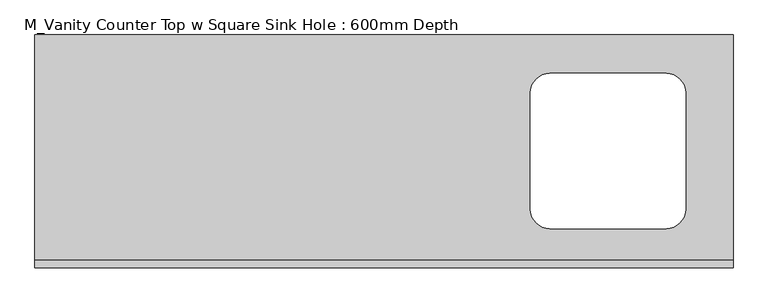
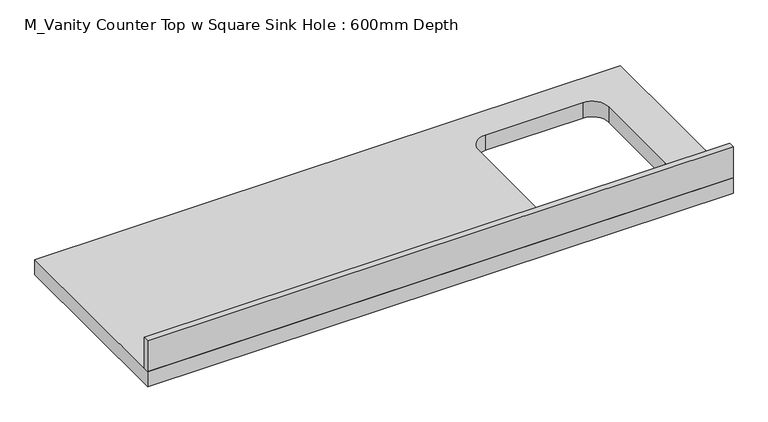
"""IFC4 building model written with IfcOpenShell, lengths in millimetres: furniture geometry, M_Vanity Counter Top w Square Sink Hole : 600mm Depth."""

from ifc_helpers import new_model, si_unit, point, frame, frame_2d, origin, place, context, project, spatial, polyline, circle_curve, trimmed, segment, composite_curve, outline, extrude, source, transform, mapped, element, save


def m_vanity_counter_top_w_square_sink_hole_600mm_depth_1391e35c(model_context):
    return source(origin(), model_context, "Body", "SweptSolid", [
        extrude(outline(polyline([(-1268.7247951, 0.0), (-1268.7247951, 19.05), (560.0752049, 19.05), (560.0752049, 0.0), (-1268.7247951, 0.0)])), frame((0.0, 0.0, 762.0), z_axis=(0.0, 0.0, 1.0), x_axis=(1.0, 0.0, 0.0)), (0.0, 0.0, 1.0), 101.6),
        extrude(outline(polyline([(560.0752049, 0.0), (-1268.7247951, 0.0), (-1268.7247951, 609.6), (560.0752049, 609.6), (560.0752049, 0.0)]), holes=[composite_curve([segment(polyline([(80.0366761, 102.3), (384.8366761, 102.3)]), True, "CONTINUOUS"), segment(trimmed(circle_curve(frame_2d((384.8366761, 153.1)), 50.8), [point((384.8366761, 102.3))], [point((435.6366761, 153.1))], True, "CARTESIAN"), True, "CONTINUOUS"), segment(polyline([(435.6366761, 153.1), (435.6366761, 457.9)]), True, "CONTINUOUS"), segment(trimmed(circle_curve(frame_2d((384.8366761, 457.9)), 50.8), [point((435.6366761, 457.9))], [point((384.8366761, 508.7))], True, "CARTESIAN"), True, "CONTINUOUS"), segment(polyline([(384.8366761, 508.7), (80.0366761, 508.7)]), True, "CONTINUOUS"), segment(trimmed(circle_curve(frame_2d((80.0366761, 457.9)), 50.8), [point((80.0366761, 508.7))], [point((29.2366761, 457.9))], True, "CARTESIAN"), True, "CONTINUOUS"), segment(polyline([(29.2366761, 457.9), (29.2366761, 153.1)]), True, "CONTINUOUS"), segment(trimmed(circle_curve(frame_2d((80.0366761, 153.1)), 50.8), [point((29.2366761, 153.1))], [point((80.0366761, 102.3))], True, "CARTESIAN"), True, "CONTINUOUS")], self_intersect=False)]), frame((0.0, 0.0, 711.2), z_axis=(0.0, 0.0, 1.0), x_axis=(1.0, 0.0, 0.0)), (0.0, 0.0, 1.0), 50.8),
    ])


if __name__ == "__main__":
    model = new_model("IFC4")
    model_context = context("Model", 3, world=origin())
    ifc_project = project(units=[si_unit("LENGTHUNIT", "METRE", prefix="MILLI")], contexts=[model_context])
    site = spatial("IfcSite", under=ifc_project)
    building = spatial("IfcBuilding", under=site)
    placement = place(None, origin())
    m_vanity_counter_top_w_square_sink_hole_600mm_depth_shape = m_vanity_counter_top_w_square_sink_hole_600mm_depth_1391e35c(model_context)
    element("IfcFurniture", 1, ObjectType="M_Vanity Counter Top w Square Sink Hole : 600mm Depth", at=placement, inside=building, context=model_context, shape_type="MappedRepresentation", body=[
        mapped(m_vanity_counter_top_w_square_sink_hole_600mm_depth_shape, transform((0.0, 0.0, 0.0), x_axis=(1.0, 0.0, 0.0), y_axis=(0.0, 1.0, 0.0), z_axis=(0.0, 0.0, 1.0))),
    ])
    save(model, "model.ifc")

# Revit data of these elements
# Project information
#   Project Issue Date = "Issue Date"
#   Project Status = "Project Status"
#   Client Name = "Owner"
#   Project Address = "Enter address here"
#   Project Name = "Office_TI_1"
#   Project Number = "Project Number"
# Type "M_Vanity Counter Top w Square Sink Hole : 600mm Depth"
#   Counter Thickness = 0' - 2"
#   Depth = 2' - 0"
#   Height = 2' - 6"
#   Length [instance default] = 3' - 11.24409"
#   Sink Location [instance default] = 1' - 11.62205"
#   Sink Location To Wall [instance default] = 0' - 4.52756"
#   Sink Opening Depth [instance default] = 1' - 5.51969"
#   Sink Opening Width [instance default] = 1' - 8"
#   Counter Top Material = none
# Element 1 (IfcFurniture, "M_Vanity Counter Top w Square Sink Hole : 600mm Depth")
#   Length = 6' - 0"
#   Sink Location = 4' - 11.10085"
#   Sink Opening Depth = 1' - 3"
#   Sink Opening Width = 1' - 3"
#   Materials on its faces: "Counter Top"
# Materials
#   "Counter Top": class "Wood", colour RGB 226 177 128, transparency 0
